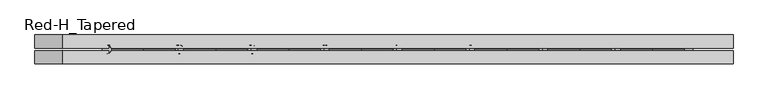
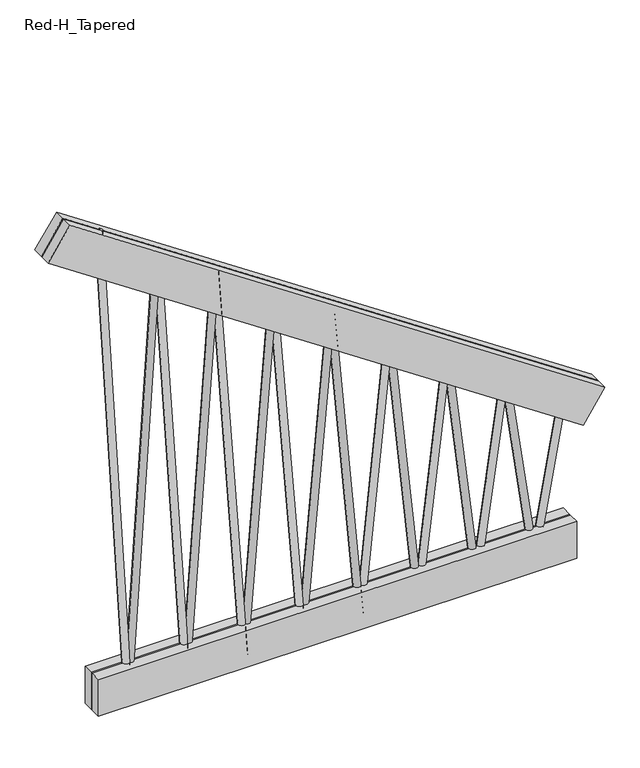
"""IFC4 building model written with IfcOpenShell, lengths in millimetres: beam geometry, Construction_Frames_RedBuilt_Openweb_Red-H_Tapered : Red-H_Tapered."""

import ifcopenshell
import ifcopenshell.guid

model = None  # the IFC model being written
_history = None  # IfcOwnerHistory: only IFC2X3 demands one
_inside = {}  # id of a spatial element -> (the spatial element, [elements in it])
_under = {}  # id of a project, library or spatial element -> (it, [spatial elements below it])
_declared = {}  # id of a project -> (the project, [libraries it declares])
_typed = {}  # id of a type object -> (the type object, [elements of that type])
_made_of = {}  # id of a material, layer set ... -> (it, [elements and type objects made of it])


def new_model(schema):
    """Start an empty IFC model of exactly this schema.

    Asked for "IFC4X3", IfcOpenShell would pick the latest addendum, in which some entities
    have other attributes; the version numbers below select the first issue.
    IFC2X3 requires an IfcOwnerHistory on every rooted entity: one is made here for all.
    """
    global model, _history
    if schema == "IFC4X3":
        model = ifcopenshell.file(schema_version=(4, 3, 0, 0))
    else:
        model = ifcopenshell.file(schema=schema)
    _inside.clear()
    _under.clear()
    _declared.clear()
    _typed.clear()
    _made_of.clear()
    _history = None
    if model.schema == "IFC2X3":
        org = make("IfcOrganization", Name="unknown")
        user = make(
            "IfcPersonAndOrganization",
            ThePerson=make("IfcPerson", FamilyName="unknown"),
            TheOrganization=org,
        )
        app = make(
            "IfcApplication",
            ApplicationDeveloper=org,
            Version="unknown",
            ApplicationFullName="unknown",
            ApplicationIdentifier="unknown",
        )
        _history = make(
            "IfcOwnerHistory",
            OwningUser=user,
            OwningApplication=app,
            ChangeAction="ADDED",
            CreationDate=0,
        )
    return model


def make(cls, **values):
    """One entity of the class cls with the attributes given. An attribute that is None is left unset."""
    return model.create_entity(
        cls, **{name: value for name, value in values.items() if value is not None}
    )


def rooted(cls, **values):
    """An entity with a GlobalId (a new one), such as an element, a storey or a relation."""
    return make(cls, GlobalId=ifcopenshell.guid.new(), OwnerHistory=_history, **values)


def si_unit(unit_type, name, prefix=None):
    """IfcSIUnit, for example si_unit("LENGTHUNIT", "METRE", prefix="MILLI")."""
    return make("IfcSIUnit", UnitType=unit_type, Prefix=prefix, Name=name)


def assignment(units):
    """IfcUnitAssignment: the units of a project."""
    return None if units is None else make("IfcUnitAssignment", Units=units)


def point(xyz):
    """IfcCartesianPoint."""
    return None if xyz is None else make("IfcCartesianPoint", Coordinates=xyz)


def direction(xyz):
    """IfcDirection."""
    return None if xyz is None else make("IfcDirection", DirectionRatios=xyz)


def frame(location, z_axis=None, x_axis=None):
    """IfcAxis2Placement3D, a coordinate frame: its origin and axes. An axis left out is left unset."""
    return make(
        "IfcAxis2Placement3D",
        Location=point(location),
        Axis=direction(z_axis),
        RefDirection=direction(x_axis),
    )


def frame_2d(location, x_axis=None):
    """IfcAxis2Placement2D, a coordinate frame in the plane: its origin and x axis."""
    return make(
        "IfcAxis2Placement2D", Location=point(location), RefDirection=direction(x_axis)
    )


def origin():
    """The frame at (0, 0, 0) with its axes left unset."""
    return frame((0.0, 0.0, 0.0))


def origin_2d():
    """The frame at (0, 0) in the plane with its x axis left unset."""
    return frame_2d((0.0, 0.0))


def place(relative_to, where):
    """IfcLocalPlacement: puts the frame where relative to a parent placement (None: the world)."""
    return make(
        "IfcLocalPlacement", PlacementRelTo=relative_to, RelativePlacement=where
    )


def context(
    kind, dimensions, precision=None, world=None, true_north=None, identifier=None
):
    """IfcGeometricRepresentationContext, for example the 3D "Model" context."""
    return make(
        "IfcGeometricRepresentationContext",
        ContextIdentifier=identifier,
        ContextType=kind,
        CoordinateSpaceDimension=dimensions,
        Precision=precision,
        WorldCoordinateSystem=world,
        TrueNorth=true_north,
    )


def project(units=None, contexts=None):
    """IfcProject with its units and contexts."""
    return rooted(
        "IfcProject",
        Name="project",
        RepresentationContexts=contexts,
        UnitsInContext=assignment(units),
    )


def spatial(cls, under=None, at=None, **own):
    """A site, building, storey or space (cls), placed at a placement, below another one or the project."""
    s = rooted(cls, ObjectPlacement=at, **own)
    if under is not None:
        _under.setdefault(under.id(), (under, []))[1].append(s)
    return s


def polyline(points):
    """IfcPolyline through the points."""
    return make("IfcPolyline", Points=[point(p) for p in points])


def circle_curve(where, radius):
    """IfcCircle in the frame where."""
    return make("IfcCircle", Position=where, Radius=radius)


def trimmed(basis, trim1, trim2, sense, master):
    """IfcTrimmedCurve: the piece of a basis curve between two trims."""
    return make(
        "IfcTrimmedCurve",
        BasisCurve=basis,
        Trim1=trim1,
        Trim2=trim2,
        SenseAgreement=sense,
        MasterRepresentation=master,
    )


def segment(curve, same_sense, transition):
    """IfcCompositeCurveSegment."""
    return make(
        "IfcCompositeCurveSegment",
        Transition=transition,
        SameSense=same_sense,
        ParentCurve=curve,
    )


def composite_curve(segments, self_intersect=None):
    """IfcCompositeCurve: segments joined end to end."""
    return make("IfcCompositeCurve", Segments=segments, SelfIntersect=self_intersect)


def outline(outer, holes=None, kind="AREA"):
    """IfcArbitraryClosedProfileDef: a profile drawn as a closed curve; with holes, ...WithVoids."""
    if holes is None:
        return make("IfcArbitraryClosedProfileDef", ProfileType=kind, OuterCurve=outer)
    return make(
        "IfcArbitraryProfileDefWithVoids",
        ProfileType=kind,
        OuterCurve=outer,
        InnerCurves=holes,
    )


def extrude(swept, where, along, depth):
    """IfcExtrudedAreaSolid: the profile swept, set in the frame where, extruded along a direction by depth."""
    return make(
        "IfcExtrudedAreaSolid",
        SweptArea=swept,
        Position=where,
        ExtrudedDirection=direction(along),
        Depth=depth,
    )


def shape(context_of_items, identifier, shape_type, items):
    """IfcShapeRepresentation: the items that make up one representation, for example the "Body"."""
    return make(
        "IfcShapeRepresentation",
        ContextOfItems=context_of_items,
        RepresentationIdentifier=identifier,
        RepresentationType=shape_type,
        Items=items,
    )


def source(mapping_origin, context_of_items, identifier, shape_type, items):
    """IfcRepresentationMap: a shape defined once, which mapped items show again and again."""
    return make(
        "IfcRepresentationMap",
        MappingOrigin=mapping_origin,
        MappedRepresentation=shape(context_of_items, identifier, shape_type, items),
    )


def transform(
    local_origin,
    x_axis=None,
    y_axis=None,
    z_axis=None,
    scale=None,
    scale2=None,
    scale3=None,
    uniform=True,
):
    """IfcCartesianTransformationOperator3D, or its non-uniform kind. x_axis, y_axis, z_axis: its Axis1, 2, 3."""
    if uniform:
        return make(
            "IfcCartesianTransformationOperator3D",
            Axis1=direction(x_axis),
            Axis2=direction(y_axis),
            LocalOrigin=point(local_origin),
            Scale=scale,
            Axis3=direction(z_axis),
        )
    return make(
        "IfcCartesianTransformationOperator3DnonUniform",
        Axis1=direction(x_axis),
        Axis2=direction(y_axis),
        LocalOrigin=point(local_origin),
        Scale=scale,
        Axis3=direction(z_axis),
        Scale2=scale2,
        Scale3=scale3,
    )


def mapped(mapping_source, mapping_target):
    """IfcMappedItem: shows the shape of a source again, moved by a transform."""
    return make(
        "IfcMappedItem", MappingSource=mapping_source, MappingTarget=mapping_target
    )


def made_of(thing, what):
    """Note that an element or type object is made of a material, layer set ...; save() writes the relation."""
    if what is not None:
        _made_of.setdefault(what.id(), (what, []))[1].append(thing)
    return thing


def element(
    cls,
    number,
    at=None,
    inside=None,
    cuts=None,
    type_object=None,
    material=None,
    context=None,
    identifier="Body",
    shape_type=None,
    held_by="IfcProductDefinitionShape",
    body=None,
    shapes=None,
    **own,
):
    """One element of the class cls, such as IfcWall. Its Tag is "e" and its number.

    at: its placement. inside: the storey or other place that contains it. cuts: it is an
    opening in that element (IfcRelVoidsElement). A single representation is given by context,
    identifier, shape_type and body (its items); several are given by shapes. held_by: the class
    of the entity that holds the representations. save() writes the other relations.
    """
    e = rooted(cls, Tag="e%d" % number, ObjectPlacement=at, **own)
    if body is not None:
        shapes = [shape(context, identifier, shape_type, body)]
    if shapes is not None:
        e.Representation = make(held_by, Representations=shapes)
    if inside is not None:
        _inside.setdefault(inside.id(), (inside, []))[1].append(e)
    if cuts is not None:
        rooted(
            "IfcRelVoidsElement", RelatingBuildingElement=cuts, RelatedOpeningElement=e
        )
    if type_object is not None:
        _typed.setdefault(type_object.id(), (type_object, []))[1].append(e)
    return made_of(e, material)


def aggregate(whole, parts):
    """IfcRelAggregates: a whole, such as a stair, and the parts it consists of."""
    return rooted("IfcRelAggregates", RelatingObject=whole, RelatedObjects=parts)


def save(model, path):
    """Write the relations noted so far, then the file.

    IfcRelAggregates (storeys below a building ...), IfcRelContainedInSpatialStructure (elements
    in a storey), IfcRelDefinesByType, IfcRelAssociatesMaterial and IfcRelDeclares: one each for
    every whole, place, type object, material and project.
    """
    for whole, parts in _under.values():
        aggregate(whole, parts)
    for where, things in _inside.values():
        rooted(
            "IfcRelContainedInSpatialStructure",
            RelatedElements=things,
            RelatingStructure=where,
        )
    for kind, things in _typed.values():
        rooted("IfcRelDefinesByType", RelatedObjects=things, RelatingType=kind)
    for what, things in _made_of.values():
        rooted("IfcRelAssociatesMaterial", RelatedObjects=things, RelatingMaterial=what)
    for by, libraries in _declared.values():
        rooted("IfcRelDeclares", RelatingContext=by, RelatedDefinitions=libraries)
    model.write(path)


def red_h_tapered_7e877e6e(model_context):
    return source(origin(), model_context, "Body", "SweptSolid", [
        extrude(outline(composite_curve([segment(trimmed(circle_curve(origin_2d(), 12.7), [point((0.0, 12.7))], [point((0.0, -12.7000001))], False, "CARTESIAN"), True, "CONTINUOUS"), segment(trimmed(circle_curve(origin_2d(), 12.7), [point((0.0, -12.7000001))], [point((0.0, 12.7))], False, "CARTESIAN"), True, "CONTINUOUS")], self_intersect=False)), frame((-103.6835937, 0.0, -367.0101562), z_axis=(-0.07752910677178004, 0.0, 0.9969900890195299), x_axis=(0.0, -1.0, 0.0)), (0.0, 0.0, 1.0), 1337.3505522),
        extrude(outline(composite_curve([segment(trimmed(circle_curve(origin_2d(), 12.7), [point((0.0, -12.7000001))], [point((0.0, 12.7))], False, "CARTESIAN"), True, "CONTINUOUS"), segment(trimmed(circle_curve(origin_2d(), 12.7), [point((0.0, 12.7))], [point((0.0, -12.7000001))], False, "CARTESIAN"), True, "CONTINUOUS")], self_intersect=False)), frame((-311.0507812, 0.0, -367.0101562), z_axis=(0.0775291067717789, 0.0, 0.9969900890195299), x_axis=(0.0, -1.0, 0.0)), (0.0, 0.0, 1.0), 1337.3505522),
        extrude(outline(composite_curve([segment(trimmed(circle_curve(origin_2d(), 12.7), [point((0.0, 12.7))], [point((0.0, -12.7000001))], False, "CARTESIAN"), True, "CONTINUOUS"), segment(trimmed(circle_curve(origin_2d(), 12.7), [point((0.0, -12.7000001))], [point((0.0, 12.7))], False, "CARTESIAN"), True, "CONTINUOUS")], self_intersect=False)), frame((-311.0507812, 0.0, -367.0101562), z_axis=(-0.06973747957372682, 0.0, 0.997565378279892), x_axis=(0.0, -1.0, 0.0)), (0.0, 0.0, 1.0), 1486.7700178),
        extrude(outline(composite_curve([segment(trimmed(circle_curve(origin_2d(), 12.7), [point((0.0, -12.7000001))], [point((0.0, 12.7))], False, "CARTESIAN"), True, "CONTINUOUS"), segment(trimmed(circle_curve(origin_2d(), 12.7), [point((0.0, 12.7))], [point((0.0, -12.7000001))], False, "CARTESIAN"), True, "CONTINUOUS")], self_intersect=False)), frame((-518.4179687, 0.0, -367.0101562), z_axis=(0.06973747957373565, 0.0, 0.9975653782798914), x_axis=(0.0, -1.0, 0.0)), (0.0, 0.0, 1.0), 1486.7700178),
        extrude(outline(composite_curve([segment(trimmed(circle_curve(origin_2d(), 12.7), [point((0.0, 12.6999999))], [point((0.0, -12.7))], False, "CARTESIAN"), True, "CONTINUOUS"), segment(trimmed(circle_curve(origin_2d(), 12.7), [point((0.0, -12.7))], [point((0.0, 12.6999999))], False, "CARTESIAN"), True, "CONTINUOUS")], self_intersect=False)), frame((-518.4179687, 0.0, -367.0101562), z_axis=(-0.06336606765698263, 0.0, 0.9979903513910797), x_axis=(0.0, -1.0, 0.0)), (0.0, 0.0, 1.0), 1636.2636595),
        extrude(outline(composite_curve([segment(trimmed(circle_curve(origin_2d(), 12.7), [point((0.0, -12.7))], [point((0.0, 12.6999999))], False, "CARTESIAN"), True, "CONTINUOUS"), segment(trimmed(circle_curve(origin_2d(), 12.7), [point((0.0, 12.6999999))], [point((0.0, -12.7))], False, "CARTESIAN"), True, "CONTINUOUS")], self_intersect=False)), frame((-725.7851562, 0.0, -367.0101562), z_axis=(0.0633660676569758, 0.0, 0.9979903513910802), x_axis=(0.0, -1.0, 0.0)), (0.0, 0.0, 1.0), 1636.2636595),
        extrude(outline(composite_curve([segment(trimmed(circle_curve(origin_2d(), 12.7), [point((0.0, 12.7))], [point((0.0, -12.7000001))], False, "CARTESIAN"), True, "CONTINUOUS"), segment(trimmed(circle_curve(origin_2d(), 12.7), [point((0.0, -12.7000001))], [point((0.0, 12.7))], False, "CARTESIAN"), True, "CONTINUOUS")], self_intersect=False)), frame((-725.7851562, 0.0, -367.0101562), z_axis=(-0.058059607877347576, 0.0, 0.9983131181814295), x_axis=(0.0, -1.0, 0.0)), (0.0, 0.0, 1.0), 1785.8128489),
        extrude(outline(composite_curve([segment(trimmed(circle_curve(origin_2d(), 12.7), [point((0.0, 12.7000001))], [point((0.0, -12.7))], False, "CARTESIAN"), True, "CONTINUOUS"), segment(trimmed(circle_curve(origin_2d(), 12.7), [point((0.0, -12.7))], [point((0.0, 12.7000001))], False, "CARTESIAN"), True, "CONTINUOUS")], self_intersect=False)), frame((725.7851562, 0.0, -367.0101562), z_axis=(0.1747487509576852, 0.0, 0.9846130580277356), x_axis=(0.0, -1.0, 0.0)), (0.0, 0.0, 1.0), 593.329527),
        extrude(outline(composite_curve([segment(trimmed(circle_curve(origin_2d(), 12.7), [point((0.0, -12.7))], [point((0.0, 12.7000001))], False, "CARTESIAN"), True, "CONTINUOUS"), segment(trimmed(circle_curve(origin_2d(), 12.7), [point((0.0, 12.7000001))], [point((0.0, -12.7))], False, "CARTESIAN"), True, "CONTINUOUS")], self_intersect=False)), frame((725.7851562, 0.0, -367.0101562), z_axis=(-0.1398650412411641, 0.0, 0.9901705763345059), x_axis=(0.0, -1.0, 0.0)), (0.0, 0.0, 1.0), 741.3117161),
        extrude(outline(composite_curve([segment(trimmed(circle_curve(origin_2d(), 12.7), [point((0.0, 12.7000001))], [point((0.0, -12.7))], False, "CARTESIAN"), True, "CONTINUOUS"), segment(trimmed(circle_curve(origin_2d(), 12.7), [point((0.0, -12.7))], [point((0.0, 12.7000001))], False, "CARTESIAN"), True, "CONTINUOUS")], self_intersect=False)), frame((518.4179687, 0.0, -367.0101562), z_axis=(0.1398650412411653, 0.0, 0.9901705763345057), x_axis=(0.0, -1.0, 0.0)), (0.0, 0.0, 1.0), 741.3117161),
        extrude(outline(composite_curve([segment(trimmed(circle_curve(origin_2d(), 12.7), [point((0.0, -12.7))], [point((0.0, 12.7))], False, "CARTESIAN"), True, "CONTINUOUS"), segment(trimmed(circle_curve(origin_2d(), 12.7), [point((0.0, 12.7))], [point((0.0, -12.7))], False, "CARTESIAN"), True, "CONTINUOUS")], self_intersect=False)), frame((518.4179687, 0.0, -367.0101562), z_axis=(-0.11651009330054839, 0.0, 0.9931895076767059), x_axis=(0.0, -1.0, 0.0)), (0.0, 0.0, 1.0), 889.9108293),
        extrude(outline(composite_curve([segment(trimmed(circle_curve(origin_2d(), 12.7), [point((0.0, 12.7000001))], [point((0.0, -12.6999999))], False, "CARTESIAN"), True, "CONTINUOUS"), segment(trimmed(circle_curve(origin_2d(), 12.7), [point((0.0, -12.6999999))], [point((0.0, 12.7000001))], False, "CARTESIAN"), True, "CONTINUOUS")], self_intersect=False)), frame((311.0507812, 0.0, -367.0101562), z_axis=(0.11651009330054864, 0.0, 0.9931895076767059), x_axis=(0.0, -1.0, 0.0)), (0.0, 0.0, 1.0), 889.9108293),
        extrude(outline(composite_curve([segment(trimmed(circle_curve(origin_2d(), 12.7), [point((0.0, -12.6999999))], [point((0.0, 12.7))], False, "CARTESIAN"), True, "CONTINUOUS"), segment(trimmed(circle_curve(origin_2d(), 12.7), [point((0.0, 12.7))], [point((0.0, -12.6999999))], False, "CARTESIAN"), True, "CONTINUOUS")], self_intersect=False)), frame((311.0507812, 0.0, -367.0101562), z_axis=(-0.09980495701504595, 0.0, 0.9950070203547434), x_axis=(0.0, -1.0, 0.0)), (0.0, 0.0, 1.0), 1038.8621653),
        extrude(outline(composite_curve([segment(trimmed(circle_curve(origin_2d(), 12.7), [point((0.0, 12.6999999))], [point((0.0, -12.7))], False, "CARTESIAN"), True, "CONTINUOUS"), segment(trimmed(circle_curve(origin_2d(), 12.7), [point((0.0, -12.7))], [point((0.0, 12.6999999))], False, "CARTESIAN"), True, "CONTINUOUS")], self_intersect=False)), frame((103.6835938, 0.0, -367.0101562), z_axis=(0.0998049570150465, 0.0, 0.9950070203547434), x_axis=(0.0, -1.0, 0.0)), (0.0, 0.0, 1.0), 1038.8621653),
        extrude(outline(composite_curve([segment(trimmed(circle_curve(origin_2d(), 12.7), [point((0.0, -12.7000001))], [point((0.0, 12.6999999))], False, "CARTESIAN"), True, "CONTINUOUS"), segment(trimmed(circle_curve(origin_2d(), 12.7), [point((0.0, 12.6999999))], [point((0.0, -12.7000001))], False, "CARTESIAN"), True, "CONTINUOUS")], self_intersect=False)), frame((103.6835938, 0.0, -367.0101562), z_axis=(-0.08727330967728768, 0.0, 0.9961844053276343), x_axis=(0.0, -1.0, 0.0)), (0.0, 0.0, 1.0), 1188.0332502),
        extrude(outline(composite_curve([segment(trimmed(circle_curve(origin_2d(), 12.7), [point((0.0, -12.7))], [point((0.0, 12.7))], False, "CARTESIAN"), True, "CONTINUOUS"), segment(trimmed(circle_curve(origin_2d(), 12.7), [point((0.0, 12.7))], [point((0.0, -12.7))], False, "CARTESIAN"), True, "CONTINUOUS")], self_intersect=False)), frame((-103.6835937, 0.0, -367.0101562), z_axis=(0.08727330967726304, 0.0, 0.9961844053276364), x_axis=(0.0, -1.0, 0.0)), (0.0, 0.0, 1.0), 1188.0332502),
        extrude(outline(polyline([(-854.86875, -41.275), (-854.86875, -3.175), (854.86875, -3.175), (854.86875, -41.275), (-854.86875, -41.275)])), frame((0.0, 0.0, -386.0601562), z_axis=(0.0, 0.0, 1.0), x_axis=(1.0, 0.0, 0.0)), (0.0, 0.0, 1.0), 139.7),
        extrude(outline(polyline([(-854.86875, 3.175), (-854.86875, 41.275), (854.86875, 41.275), (854.86875, 3.175), (-854.86875, 3.175)])), frame((0.0, 0.0, -386.0601562), z_axis=(0.0, 0.0, 1.0), x_axis=(1.0, 0.0, 0.0)), (0.0, 0.0, 1.0), 139.7),
        extrude(outline(polyline([(0.0, -38.1), (0.0, 0.0), (2303.1824003, 0.0), (2303.1824003, -38.1), (0.0, -38.1)])), frame((-1034.2711811, -3.175, 1390.2102281), z_axis=(0.5569250615368141, 0.0, 0.8305627464750728), x_axis=(0.8305627464750728, 0.0, -0.5569250615368141)), (0.0, 0.0, 1.0), 139.7),
        extrude(outline(polyline([(0.0, -38.1), (0.0, 0.0), (2303.1824003, 0.0), (2303.1824003, -38.1), (0.0, -38.1)])), frame((-1034.2711811, 41.275, 1390.2102281), z_axis=(0.5569250615368141, 0.0, 0.8305627464750728), x_axis=(0.8305627464750728, 0.0, -0.5569250615368141)), (0.0, 0.0, 1.0), 139.7),
    ])


if __name__ == "__main__":
    model = new_model("IFC4")
    model_context = context("Model", 3, world=origin())
    ifc_project = project(units=[si_unit("LENGTHUNIT", "METRE", prefix="MILLI")], contexts=[model_context])
    site = spatial("IfcSite", under=ifc_project)
    building = spatial("IfcBuilding", under=site)
    placement = place(None, origin())
    red_h_tapered_shape = red_h_tapered_7e877e6e(model_context)
    element("IfcBeam", 1, ObjectType="Construction_Frames_RedBuilt_Openweb_Red-H_Tapered : Red-H_Tapered", at=placement, inside=building, context=model_context, shape_type="MappedRepresentation", body=[
        mapped(red_h_tapered_shape, transform((0.0, 0.0, 0.0), x_axis=(1.0, 0.0, 0.0), y_axis=(0.0, 1.0, 0.0), z_axis=(0.0, 0.0, 1.0))),
    ])
    save(model, "model.ifc")

# Revit data of these elements
# Type "Construction_Frames_RedBuilt_Openweb_Red-H_Tapered : Red-H_Tapered"
#   Youtube clip = ""
#   Weight Net (Kg) = "0"
#   Webs = "Up to 2\" diameter tubular steel"
#   Uniformat II Description = ""
#   Uniformat II Code = ""
#   Uniclass 2015 Name = "Softwood trusses"
#   Uniclass 2015 Code = "Pr_20_85_90_81"
#   Uniclass 2.0 Description = "Structural Framing Systems"
#   Uniclass 2.0 Code = "SS-15-10-75"
#   Uniclass 1.4 Description = "Trusses"
#   Uniclass 1.4 Code = "L3523"
#   UNSPSC Code = "30103606"
#   Technical description = "http://www.redbuilt.com/reference/literature-and-other-resources"
#   Region South America = "None"
#   Region Oceania = "None"
#   Region North America = "US"
#   Region Middle East = "None"
#   Region Europe = "None"
#   Region Asia = "None"
#   Region Antarctica = "None"
#   Region Africa = "None"
#   QR code = "http://bimobject.com/redbuilt/product/redbuilt-0003"
#   Product url = "http://www.redbuilt.com/products/default.aspx?id=2"
#   Product group = "Wood Trusses"
#   Product family = "Construction"
#   Product data url = "https://bimobject.com/redbuilt/product/redbuilt-0003"
#   Product certification = ""
#   Product SKU = "redbuilt-0003"
#   Product Page URL = "http://www.redbuilt.com/commercial-systems/red-m-red-h-open-web-trusses"
#   Product Guid = "2c5793f2-6ffb-4665-b825-cf90c048e711"
#   Product Documentation Link = "http://www.redbuilt.com/documents/OW_Guide_2017_07_LowRes_wLinks.pdf"
#   OmniClass Description = "Wood Trusses"
#   OmniClass Code = "23-13 35 19 13 17"
#   NBS Reference Description = ""
#   NBS Reference Code = ""
#   Material secondary = "Steel"
#   Material main = "Wood"
#   Masterformat 2014 Description = "Metal-Web Wood Joists"
#   Masterformat 2014 Code = "06 17 36"
#   Manufacturer name = "RedBuilt"
#   Manufacturer country = "United States"
#   Installation instructions = "http://www.redbuilt.com/documents/Installation_Sheets_Open-Web.pdf"
#   IFC Classification = ""
#   EAN code = ""
#   Design country = "United States"
#   Product Information = "http://redbuilt.com/products/default.aspx?id=2"
#   Model = "Red-H-Tapered"
#   Manufacturer URL = "http://redbuilt.com/"
#   Manufacturer = "RedBuilt™"
#   Description = "Open Web Truss"
#   Date of publishing = "8/17/2010"
#   Contact us = "http://redbuilt.com/contact/"
#   Chords = "Double 1½\" x 5½\" MSR lumber"
#   COBIe Type Category = ""
#   Brand url = "http://www.redbuilt.com"
#   BIMobject main category code = "construction"
#   BIMobject main category = "Construction"
#   BIMobject category code = "construction-frames-trusses"
#   BIMobject category = "Frames & Trusses"
#   Web Radius = 0' - 0 1/2"
#   Web Layout Offset Start [instance default] = 0' - 5"
#   Web Layout Offset End [instance default] = 0' - 5"
#   Web Diameter = 0' - 1"
#   TotalLength [instance default] = 20' - 0"
#   Span Minimum = 4' - 0"
#   Span Maximum = 70' - 0"
#   Span Limit [instance default] = 20' - 0"
#   Nominal width = 0' - 0"
#   Nominal height = 0' - 0"
#   Inner Depth Top [instance default] = 0' - 2.76372"
#   Depth Start [instance default] = 6' - 0"
#   Top Chord Length [instance default] = 20' - 1.19701"
#   TC Extension Start Aux [instance default] = 0' - 0"
#   TC Extension End Aux [instance default] = 0' - 0"
#   T-B Chord Length Difference L [instance default] = 0' - 4"
#   T-B Chord Length Difference [instance default] = 0' - 4"
#   Height 2 [instance default] = 6' - 0"
#   Depth Minimum at Wall = 2' - 0"
#   Depth Maximum at Wall = 6' - 0"
#   Depth Lower End [instance default] = 2' - 0"
#   Depth Higher End [instance default] = 6' - 0"
#   Depth End [instance default] = 2' - 0"
#   Depth 2 [instance default] = 2' - 0"
#   Chord Width = 0' - 3 1/4"
#   Chord Thickness = 0' - 1 1/2"
#   Chord Depth = 0' - 5 1/2"
#   Offset Start [instance default] = 0' - 0"
#   TC Extension Start [instance default] = 0' - 0"
#   End Panel = 0' - 5"
#   Offset End [instance default] = 0' - 0"
#   TC Extension End [instance default] = 0' - 0"
#   Length [instance default] = 20' - 0"
#   Angle [instance default] = 5.71059°
#   Span Limit Warning [instance default] = no
#   Edition number = 1
#   Top Bearing Start [instance default] = yes
#   Top Bearing End [instance default] = yes
#   Bottom Bearing Start [instance default] = no
#   Bottom Bearing End [instance default] = no
#   8 Panels [instance default] = yes
#   16 Panels [instance default] = no
#   12 Panels [instance default] = no
#   Web Material = RedBuilt-Steel, Galvanized
#   Clip Material = RedBuilt-Steel, Galvanized
#   Chords Material = RedBuilt-MSR
#   URL = ""
#   Assembly Code = ""
# Element 1 (IfcBeam, "Construction_Frames_RedBuilt_Openweb_Red-H_Tapered : Red-H_Tapered")
#   TotalLength = 6' - 3 5/16"
#   Span Limit = 6' - 3 5/16"
#   Inner Depth Top = 0' - 3.31101"
#   Top Chord Length = 7' - 6.67647"
#   Depth 2 = 4' - 2 1/2"
#   Angle = 33.8434°
#   Materials on its faces: "RedBuilt-Steel, Galvanized", "RedBuilt-MSR"
# Materials
#   "RedBuilt-Steel, Galvanized": class "Metal", colour RGB 164 172 176, transparency 0, Manufacturer = "RedBuilt. LLC", Comments = "Openweb Metal Web", URL = "http://www.redbuilt.com/", Description = "Galvanized steel", Cost = 0
#   "RedBuilt-MSR": class "Wood", colour RGB 213 182 136, transparency 0, Manufacturer = "RedBuilt, LLC", URL = "http://www.redbuilt.com/", Cost = 0
